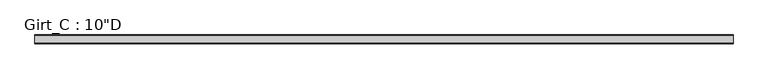
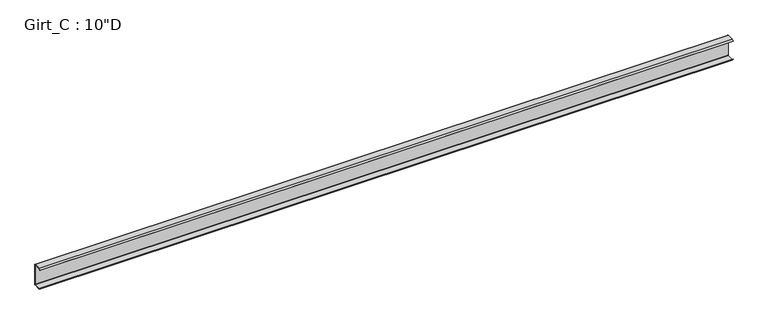
"""IFC4 building model written with IfcOpenShell, lengths in millimetres: beam geometry."""

from ifc_helpers import new_model, si_unit, point, frame, frame_2d, origin, place, context, project, spatial, polyline, circle_curve, trimmed, segment, composite_curve, outline, extrude, source, transform, mapped, element, save


def beam_0a52ee2c(model_context):
    return source(origin(), model_context, "Body", "SweptSolid", [
        extrude(outline(composite_curve([segment(polyline([(-87.5109375, 127.0), (-3.3734375, 127.0)]), True, "CONTINUOUS"), segment(trimmed(circle_curve(frame_2d((-3.3734375, 122.2375)), 4.7625), [point((-3.3734375, 127.0))], [point((1.3890625, 122.2375))], False, "CARTESIAN"), True, "CONTINUOUS"), segment(polyline([(1.3890625, 122.2375), (1.3890625, -122.2375)]), True, "CONTINUOUS"), segment(trimmed(circle_curve(frame_2d((-3.3734375, -122.2375)), 4.7625), [point((1.3890625, -122.2375))], [point((-3.3734375, -127.0))], False, "CARTESIAN"), True, "CONTINUOUS"), segment(polyline([(-3.3734375, -127.0), (-87.5109375, -127.0), (-99.7792647, -112.379177), (-97.6510975, -110.5934327), (-86.2154765, -124.221875), (-3.2694106, -124.221875)]), True, "CONTINUOUS"), segment(trimmed(circle_curve(frame_2d((-3.3748024, -122.2389339)), 1.9857399), [point((-3.2694106, -124.221875))], [point((-1.3890625, -122.2389339))], True, "CARTESIAN"), True, "CONTINUOUS"), segment(polyline([(-1.3890625, -122.2389339), (-1.3890625, 122.2381931)]), True, "CONTINUOUS"), segment(trimmed(circle_curve(frame_2d((-3.3741066, 122.2381931)), 1.9850441), [point((-1.3890625, 122.2381931))], [point((-3.3005807, 124.221875))], True, "CARTESIAN"), True, "CONTINUOUS"), segment(polyline([(-3.3005807, 124.221875), (-86.2154765, 124.221875), (-97.6278742, 110.621109), (-99.7560415, 112.4068534), (-87.5109375, 127.0)]), True, "CONTINUOUS")], self_intersect=False)), frame((-4028.694, 0.0, 0.0), z_axis=(1.0, 0.0, 0.0), x_axis=(0.0, 1.0, 0.0)), (0.0, 0.0, 1.0), 8044.688),
    ])


if __name__ == "__main__":
    model = new_model("IFC4")
    model_context = context("Model", 3, world=origin())
    ifc_project = project(units=[si_unit("LENGTHUNIT", "METRE", prefix="MILLI")], contexts=[model_context])
    site = spatial("IfcSite", under=ifc_project)
    building = spatial("IfcBuilding", under=site)
    placement = place(None, origin())
    beam_shape = beam_0a52ee2c(model_context)
    element("IfcBeam", 1, ObjectType="Girt_C : 10\"D", at=placement, inside=building, context=model_context, shape_type="MappedRepresentation", body=[
        mapped(beam_shape, transform((0.0, 0.0, 0.0), x_axis=(1.0, 0.0, 0.0), y_axis=(0.0, 1.0, 0.0), z_axis=(0.0, 0.0, 1.0))),
    ])
    save(model, "model.ifc")

# Revit data of these elements
# Type "Girt_C : 10\"D"
#   half leg = 0' - 1 3/4"
#   Web_Thickness = 0' - 0 7/64"
#   Length [instance default] = 10' - 0"
#   Leg_1 = 0' - 3 1/2"
#   Height = 0' - 10"
#   Structural Material [instance default] = none
# Element 1 (IfcBeam, "Girt_C : 10\"D")
#   Structural Material = STRUCTURAL STEEL - SEE STRUCT. DWGS
#   Materials on its faces: "STRUCTURAL STEEL - SEE STRUCT. DWGS"
# Materials
#   "STRUCTURAL STEEL - SEE STRUCT. DWGS": class "Metal", colour RGB 137 146 153, transparency 0, Description = "Steel, mill finish", Cost = 0
